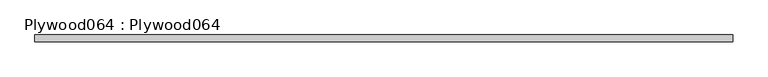
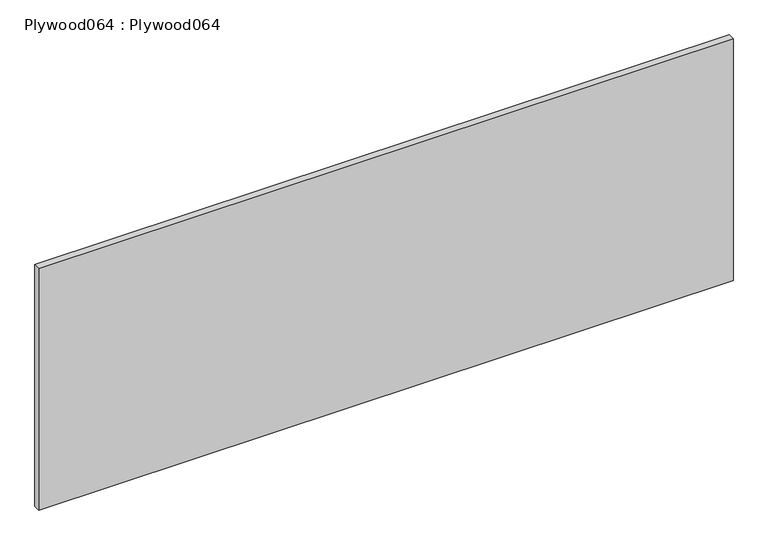
"""IFC4 building model written with IfcOpenShell, lengths in millimetres: proxy geometry, Plywood064 : Plywood064."""

from ifc_helpers import new_model, si_unit, frame, origin, place, context, project, spatial, polyline, outline, extrude, source, transform, mapped, element, save


def plywood064_plywood064_662705af(model_context):
    return source(origin(), model_context, "Body", "SweptSolid", [
        extrude(outline(polyline([(14383.0178845, -4637.5425368), (14383.0178845, -4656.5925368), (12383.0178845, -4656.5925368), (12383.0178845, -4637.5425368), (14383.0178845, -4637.5425368)])), frame((0.0, 0.0, 39020.496), z_axis=(0.0, 0.0, 1.0), x_axis=(1.0, 0.0, 0.0)), (0.0, 0.0, 1.0), 736.6),
    ])


if __name__ == "__main__":
    model = new_model("IFC4")
    model_context = context("Model", 3, world=origin())
    ifc_project = project(units=[si_unit("LENGTHUNIT", "METRE", prefix="MILLI")], contexts=[model_context])
    site = spatial("IfcSite", under=ifc_project)
    building = spatial("IfcBuilding", under=site)
    placement = place(None, origin())
    plywood064_plywood064_shape = plywood064_plywood064_662705af(model_context)
    element("IfcBuildingElementProxy", 1, Name="Plywood064 : Plywood064", ObjectType="Plywood064 : Plywood064", at=placement, inside=building, context=model_context, shape_type="MappedRepresentation", body=[
        mapped(plywood064_plywood064_shape, transform((0.0, 0.0, 0.0), x_axis=(1.0, 0.0, 0.0), y_axis=(0.0, 1.0, 0.0), z_axis=(0.0, 0.0, 1.0))),
    ])
    save(model, "model.ifc")

# Revit data of these elements
# Type "Plywood064 : Plywood064"
#   NameOverride = "Plywood064"
# Element 1 (IfcBuildingElementProxy, "Plywood064 : Plywood064")
#   Materials on its faces: "CDX PLYWOOD - SEE STRUCTURAL DWGS"
# Materials
#   "CDX PLYWOOD - SEE STRUCTURAL DWGS": class "Unassigned", colour RGB 177 130 114, transparency 0, Cost = 0
